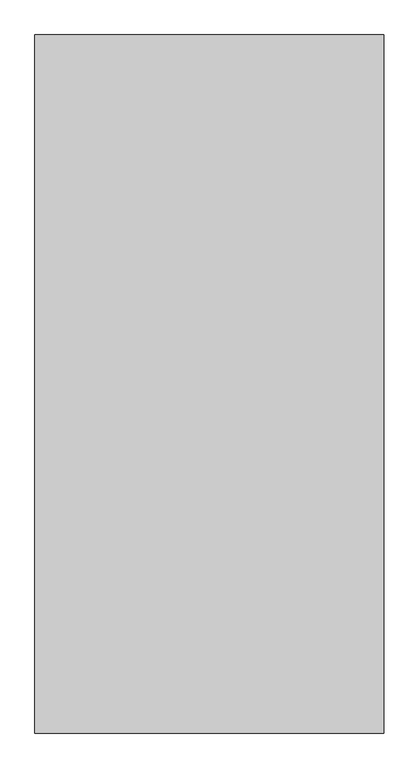
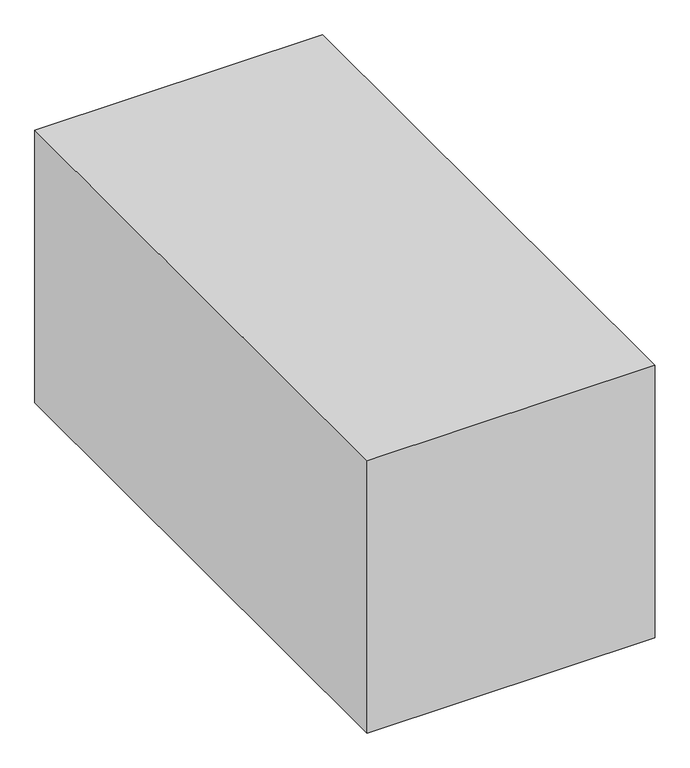
"""IFC4 building model written with IfcOpenShell, lengths in millimetres: proxy geometry, Space Planning Box_hec : Space Planning Box_hec."""

from ifc_helpers import new_model, si_unit, origin, origin_with_axes, place, context, project, spatial, polyline, outline, extrude, source, transform, mapped, element, save


def generic_models_43059f4e(model_context):
    return source(origin(), model_context, "Body", "SweptSolid", [
        extrude(outline(polyline([(3000.0, 6000.0), (3000.0, -6000.0), (-3000.0, -6000.0), (-3000.0, 6000.0), (3000.0, 6000.0)])), origin_with_axes(), (0.0, 0.0, 1.0), 6000.0),
    ])


if __name__ == "__main__":
    model = new_model("IFC4")
    model_context = context("Model", 3, world=origin())
    ifc_project = project(units=[si_unit("LENGTHUNIT", "METRE", prefix="MILLI")], contexts=[model_context])
    site = spatial("IfcSite", under=ifc_project)
    building = spatial("IfcBuilding", under=site)
    placement = place(None, origin())
    generic_models_shape = generic_models_43059f4e(model_context)
    element("IfcBuildingElementProxy", 1, Name="Space Planning Box_hec : Space Planning Box_hec", ObjectType="Space Planning Box_hec : Space Planning Box_hec", at=placement, inside=building, context=model_context, shape_type="MappedRepresentation", body=[
        mapped(generic_models_shape, transform((0.0, 0.0, 0.0), x_axis=(1.0, 0.0, 0.0), y_axis=(0.0, 1.0, 0.0), z_axis=(0.0, 0.0, 1.0))),
    ])
    save(model, "model.ifc")

# Revit data of these elements
# Type "Space Planning Box_hec : Space Planning Box_hec"
#   Type Comments = "..."
#   Room Name [instance default] = "?"
#   Interior Finish [instance default] = ""
#   Exterior Finish [instance default] = ""
#   Department [instance default] = ""
#   Assembly Code = "..."
#   Width [instance default] = 1524 mm
#   Program Area [instance default] = 0.00 m²
#   Length [instance default] = 1524 mm
#   Height [instance default] = 1524 mm
#   Area [instance default] = 2.32258 m²
#   Fill Color [instance default] = Cyan
#   Default Elevation = 0
# Element 1 (IfcBuildingElementProxy, "Space Planning Box_hec : Space Planning Box_hec")
#   Room Name = "Toilet (M)"
#   Interior Finish = "IF5"
#   Exterior Finish = "EF1"
#   Department = "AR"
#   Width = 6000 mm
#   Program Area = 72.00 m²
#   Length = 12000 mm
#   Height = 6000 mm
#   Area = 72.00 m²
#   Materials on its faces: "Cyan"
# Materials
#   "Cyan": class "Generic", colour RGB 0 255 255, transparency 0.2, Cost = 0
